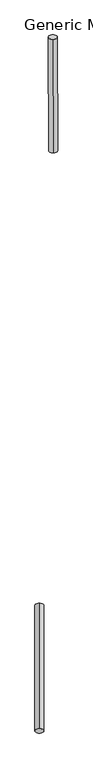
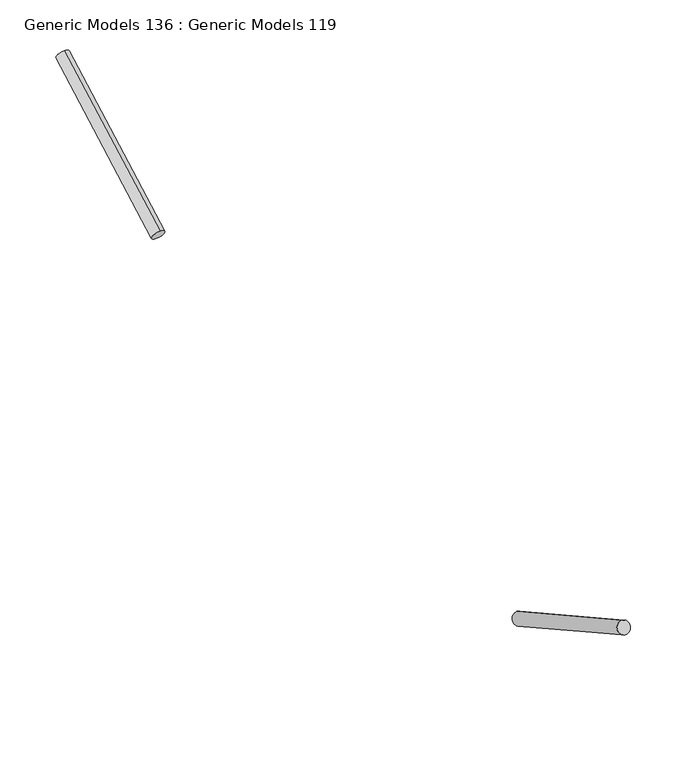
"""IFC4 building model written with IfcOpenShell, lengths in millimetres: proxy geometry, Generic Models 136 : Generic Models 119."""

from ifc_helpers import new_model, si_unit, point, frame, origin, place, context, project, spatial, circle_curve, trimmed, source, transform, mapped, element, save
from ifc_brep_helpers import plane_surface, extruded_surface, advanced_brep


def generic_models_136_generic_models_119_0a16d049(model_context):
    return source(origin(), model_context, "Body", "AdvancedBrep", [
        advanced_brep(
        [(32003.9965778, 33985.848725, 270966.7195484), (32003.9965778, 34004.3199716, 270933.3965376), (32002.4450787, 34469.0323822, 271234.5526231), (32002.4450787, 34487.5036288, 271201.2296123)],
        [
            (0, 1, circle_curve(frame((32003.9965778, 33995.0843483, 270950.058043), z_axis=(0.0, -0.8746197071393959, -0.4848096202463367), x_axis=(0.0, 0.4848096202463367, -0.8746197071393959)), 19.05)),
            (1, 0, circle_curve(frame((32003.9965778, 33995.0843483, 270950.058043), z_axis=(0.0, -0.8746197071393959, -0.4848096202463367), x_axis=(0.0, 0.4848096202463367, -0.8746197071393959)), 19.05)),
            (2, 3, circle_curve(frame((32002.4450787, 34478.2680055, 271217.8911177), z_axis=(0.0, 0.8746197071393959, 0.4848096202463367), x_axis=(0.0, 0.4848096202463367, -0.8746197071393959)), 19.05)),
            (3, 2, circle_curve(frame((32002.4450787, 34478.2680055, 271217.8911177), z_axis=(0.0, 0.8746197071393959, 0.4848096202463367), x_axis=(0.0, 0.4848096202463367, -0.8746197071393959)), 19.05)),
            (0, 2),
            (3, 1),
        ],
        [
            plane_surface(frame((32003.9965778, 33995.0843483, 270950.058043), z_axis=(0.0, -0.874619707139396, -0.4848096202463368), x_axis=(-1.0, 0.0, 0.0))),
            plane_surface(frame((32002.4450787, 34478.2680055, 271217.8911177), z_axis=(0.0, 0.874619707139396, 0.4848096202463368), x_axis=(-1.0, 0.0, 0.0))),
            extruded_surface(trimmed(circle_curve(frame((32002.4450787, 34478.2680055, 271217.8911177), z_axis=(0.0, -0.8746197071393959, -0.4848096202463367), x_axis=(0.0, 0.4848096202463367, -0.8746197071393959)), 19.05), [point((32002.4450787, 34469.0323822, 271234.5526231))], [point((32002.4450787, 34487.5036288, 271201.2296123))], True, "CARTESIAN"), (1.55149910000182, -483.1836572000029, -267.8330747000291), 552.452178598201),
            extruded_surface(trimmed(circle_curve(frame((32002.4450787, 34478.2680055, 271217.8911177), z_axis=(0.0, -0.8746197071393959, -0.4848096202463367), x_axis=(0.0, 0.4848096202463367, -0.8746197071393959)), 19.05), [point((32002.4450787, 34487.5036288, 271201.2296123))], [point((32002.4450787, 34469.0323822, 271234.5526231))], True, "CARTESIAN"), (1.55149910000182, -483.1836572000029, -267.8330747000291), 552.452178598201),
        ],
        [
            (0, [[1, 2]]),
            (1, [[3, 4]]),
            (2, [[-1, 5, -4, 6]]),
            (3, [[-2, -6, -3, -5]]),
        ],
    ),
        advanced_brep(
        [(31945.3483901, 32051.1312525, 270936.4750786), (31945.3483901, 32069.602499, 270969.7980895), (31945.2937775, 31517.963079, 271232.0150231), (31945.2937775, 31536.4343255, 271265.338034)],
        [
            (0, 1, circle_curve(frame((31945.3483901, 32060.3668758, 270953.1365841), z_axis=(0.0, 0.874619707139394, -0.48480962024634044), x_axis=(0.0, 0.48480962024634044, 0.874619707139394)), 19.05)),
            (1, 0, circle_curve(frame((31945.3483901, 32060.3668758, 270953.1365841), z_axis=(0.0, 0.874619707139394, -0.48480962024634044), x_axis=(0.0, 0.48480962024634044, 0.874619707139394)), 19.05)),
            (2, 3, circle_curve(frame((31945.2937775, 31527.1987023, 271248.6765286), z_axis=(0.0, -0.874619707139394, 0.48480962024634044), x_axis=(0.0, 0.48480962024634044, 0.874619707139394)), 19.05)),
            (3, 2, circle_curve(frame((31945.2937775, 31527.1987023, 271248.6765286), z_axis=(0.0, -0.874619707139394, 0.48480962024634044), x_axis=(0.0, 0.48480962024634044, 0.874619707139394)), 19.05)),
            (0, 2),
            (3, 1),
        ],
        [
            plane_surface(frame((31945.3483901, 32060.3668758, 270953.1365841), z_axis=(0.0, 0.874619707139394, -0.48480962024634044), x_axis=(-1.0, 0.0, 0.0))),
            plane_surface(frame((31945.2937775, 31527.1987023, 271248.6765286), z_axis=(0.0, -0.874619707139394, 0.48480962024634044), x_axis=(-1.0, 0.0, 0.0))),
            extruded_surface(trimmed(circle_curve(frame((31945.2937775, 31527.1987023, 271248.6765286), z_axis=(0.0, 0.874619707139394, -0.48480962024634044), x_axis=(0.0, 0.48480962024634044, 0.874619707139394)), 19.05), [point((31945.2937775, 31517.963079, 271232.0150231))], [point((31945.2937775, 31536.4343255, 271265.338034))], True, "CARTESIAN"), (0.05461260000083712, 533.1681734999984, -295.5399444999639), 609.600002469572),
            extruded_surface(trimmed(circle_curve(frame((31945.2937775, 31527.1987023, 271248.6765286), z_axis=(0.0, 0.874619707139394, -0.48480962024634044), x_axis=(0.0, 0.48480962024634044, 0.874619707139394)), 19.05), [point((31945.2937775, 31536.4343255, 271265.338034))], [point((31945.2937775, 31517.963079, 271232.0150231))], True, "CARTESIAN"), (0.05461260000083712, 533.1681734999984, -295.5399444999639), 609.600002469572),
        ],
        [
            (0, [[1, 2]]),
            (1, [[3, 4]]),
            (2, [[-1, 5, -4, 6]]),
            (3, [[-2, -6, -3, -5]]),
        ],
    ),
    ])


if __name__ == "__main__":
    model = new_model("IFC4")
    model_context = context("Model", 3, world=origin())
    ifc_project = project(units=[si_unit("LENGTHUNIT", "METRE", prefix="MILLI")], contexts=[model_context])
    site = spatial("IfcSite", under=ifc_project)
    building = spatial("IfcBuilding", under=site)
    placement = place(None, origin())
    generic_models_136_generic_models_119_shape = generic_models_136_generic_models_119_0a16d049(model_context)
    element("IfcBuildingElementProxy", 1, Name="Generic Models 136 : Generic Models 119", ObjectType="Generic Models 136 : Generic Models 119", at=placement, inside=building, context=model_context, shape_type="MappedRepresentation", body=[
        mapped(generic_models_136_generic_models_119_shape, transform((0.0, 0.0, 0.0), x_axis=(1.0, 0.0, 0.0), y_axis=(0.0, 1.0, 0.0), z_axis=(0.0, 0.0, 1.0))),
    ])
    save(model, "model.ifc")

# Revit data of these elements
# Element 1 (IfcBuildingElementProxy, "Generic Models 136 : Generic Models 119")
#   Materials on its faces: "TURN BUCKLE"
# Materials
#   "TURN BUCKLE": class "Metal", colour RGB 199 199 199, transparency 0, Description = "Carbon steel", Cost = 0
